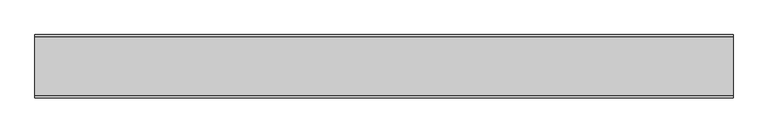
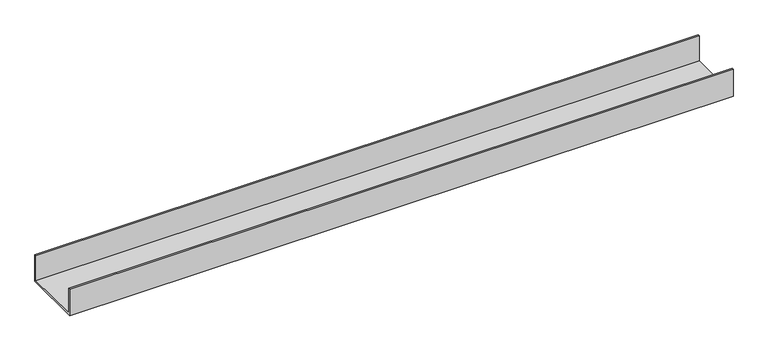
"""IFC4 building model written with IfcOpenShell, lengths in millimetres: proxy geometry, Generic Models 3:Generic Models 1:6:Generic Models 1:6 : Generic Models 3:Generic Models 1:300625:350611:Generic Models 1:6:Generic Models 1:6 : Generic Models 3:Generic Models 1:300625:350611 : Generic Models 3:Generic Models 1:6:Generic Models 1:6 : Generic Models 3:Generic Models 1:300625:350611:10 : Generic Models 3:Generic Models 1:6:Generic Models 1:6 : Generic Models 3:Generic Models 1:300625:350611:Generic Models 1:6:Generic Models 1:6 : Generic Models 3:Generic Models 1:300625:350611 : Generic Models 3:Generic Models 1:6:Generic Models 1:6 : Generic Models 3:Generic Models 1:300625:350611:301824."""

from ifc_helpers import new_model, si_unit, frame, origin, place, context, project, spatial, polyline, outline, extrude, source, transform, mapped, element, save


def generic_models_4023f549(model_context):
    return source(origin(), model_context, "Body", "SweptSolid", [
        extrude(outline(polyline([(0.0, 0.0), (95.25, 0.0), (95.25, -6.35), (6.35, -6.35), (6.35, -196.85), (95.25, -196.85), (95.25, -203.2), (0.0, -203.2), (0.0, 0.0)])), frame((573106.936724, -530848.6413842, 0.0), z_axis=(1.0, -5.345279774360279e-12, 0.0), x_axis=(0.0, 0.0, 1.0)), (0.0, 0.0, 1.0), 2241.55),
    ])


if __name__ == "__main__":
    model = new_model("IFC4")
    model_context = context("Model", 3, world=origin())
    ifc_project = project(units=[si_unit("LENGTHUNIT", "METRE", prefix="MILLI")], contexts=[model_context])
    site = spatial("IfcSite", under=ifc_project)
    building = spatial("IfcBuilding", under=site)
    placement = place(None, origin())
    generic_models_shape = generic_models_4023f549(model_context)
    element("IfcBuildingElementProxy", 1, Name="Generic Models 3:Generic Models 1:6:Generic Models 1:6 : Generic Models 3:Generic Models 1:300625:350611:Generic Models 1:6:Generic Models 1:6 : Generic Models 3:Generic Models 1:300625:350611 : Generic Models 3:Generic Models 1:6:Generic Models 1:6 : Generic Models 3:Generic Models 1:300625:350611:10 : Generic Models 3:Generic Models 1:6:Generic Models 1:6 : Generic Models 3:Generic Models 1:300625:350611:Generic Models 1:6:Generic Models 1:6 : Generic Models 3:Generic Models 1:300625:350611 : Generic Models 3:Generic Models 1:6:Generic Models 1:6 : Generic Models 3:Generic Models 1:300625:350611:301824", ObjectType="Generic Models 3:Generic Models 1:6:Generic Models 1:6 : Generic Models 3:Generic Models 1:300625:350611:Generic Models 1:6:Generic Models 1:6 : Generic Models 3:Generic Models 1:300625:350611 : Generic Models 3:Generic Models 1:6:Generic Models 1:6 : Generic Models 3:Generic Models 1:300625:350611:10 : Generic Models 3:Generic Models 1:6:Generic Models 1:6 : Generic Models 3:Generic Models 1:300625:350611:Generic Models 1:6:Generic Models 1:6 : Generic Models 3:Generic Models 1:300625:350611 : Generic Models 3:Generic Models 1:6:Generic Models 1:6 : Generic Models 3:Generic Models 1:300625:350611:301824", at=placement, inside=building, context=model_context, shape_type="MappedRepresentation", body=[
        mapped(generic_models_shape, transform((0.0, 0.0, 0.0), x_axis=(1.0, 0.0, 0.0), y_axis=(0.0, 1.0, 0.0), z_axis=(0.0, 0.0, 1.0))),
    ])
    save(model, "model.ifc")

# Revit data of these elements
# Type "Generic Models 3:Generic Models 1:6:Generic Models 1:6 : Generic Models 3:Generic Models 1:300625:350611:Generic Models 1:6:Generic Models 1:6 : Generic Models 3:Generic Models 1:300625:350611 : Generic Models 3:Generic Models 1:6:Generic Models 1:6 : Generic Models 3:Generic Models 1:300625:350611:10 : Generic Models 3:Generic Models 1:6:Generic Models 1:6 : Generic Models 3:Generic Models 1:300625:350611:Generic Models 1:6:Generic Models 1:6 : Generic Models 3:Generic Models 1:300625:350611 : Generic Models 3:Generic Models 1:6:Generic Models 1:6 : Generic Models 3:Generic Models 1:300625:350611:301824"
#   NameOverride = "Generic Models 3:Generic Models 1:6:Generic Models 1:6 : Generic Models 3:Generic Models 1:300625:350611:Generic Models 1:6:Generic Models 1:6 : Generic Models 3:Generic Models 1:300625:350611 : Generic Models 3:Generic Models 1:6:Generic Models 1:6 : Generic Models 3:Generic Models 1:300625:350611:301824"
#   ObjectTypeOverride = "Generic Models 1:6:Generic Models 1:6 : Generic Models 3:Generic Models 1:300625:350611 : Generic Models 3:Generic Models 1:6:Generic Models 1:6 : Generic Models 3:Generic Models 1:300625:350611"
#   Reference = "Generic Models 1"
#   Tag = "301824"
